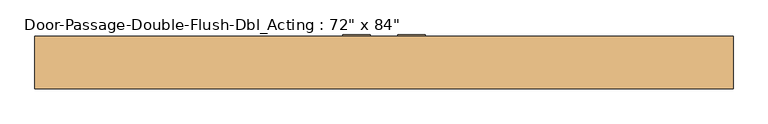
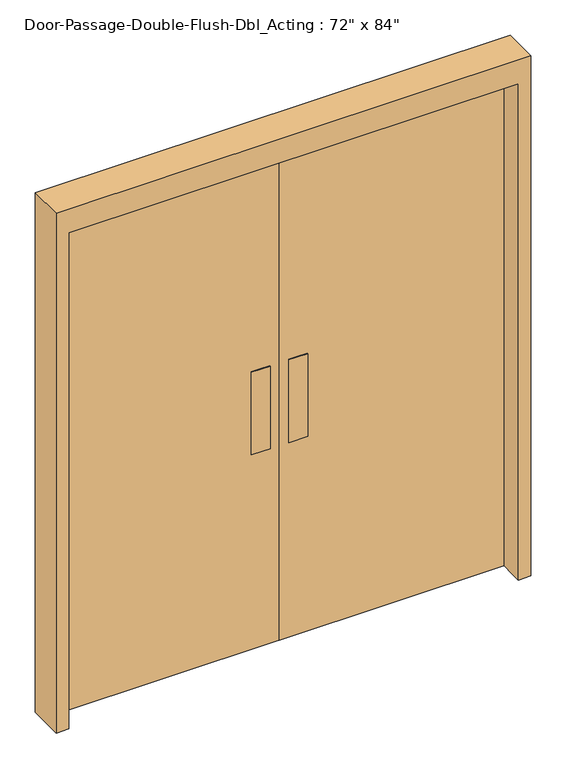
"""IFC4 building model written with IfcOpenShell, lengths in millimetres: door geometry."""

from ifc_helpers import new_model, si_unit, frame, origin, origin_with_axes, place, context, project, spatial, polyline, outline, extrude, source, transform, mapped, element, save


def door_d44e9ae0(model_context):
    return source(origin(), model_context, "Body", "SweptSolid", [
        extrude(outline(polyline([(-38.1, 34.925), (-114.3, 34.925), (-114.3, 38.1), (-38.1, 38.1), (-38.1, 34.925)])), frame((0.0, 0.0, 838.2), z_axis=(0.0, 0.0, 1.0), x_axis=(1.0, 0.0, 0.0)), (0.0, 0.0, 1.0), 355.6),
        extrude(outline(polyline([(-38.1, 85.725), (-38.1, 82.55), (-114.3, 82.55), (-114.3, 85.725), (-38.1, 85.725)])), frame((0.0, 0.0, 838.2), z_axis=(0.0, 0.0, 1.0), x_axis=(1.0, 0.0, 0.0)), (0.0, 0.0, 1.0), 355.6),
        extrude(outline(polyline([(38.1, 34.925), (38.1, 38.1), (114.3, 38.1), (114.3, 34.925), (38.1, 34.925)])), frame((0.0, 0.0, 838.2), z_axis=(0.0, 0.0, 1.0), x_axis=(1.0, 0.0, 0.0)), (0.0, 0.0, 1.0), 355.6),
        extrude(outline(polyline([(38.1, 85.725), (114.3, 85.725), (114.3, 82.55), (38.1, 82.55), (38.1, 85.725)])), frame((0.0, 0.0, 838.2), z_axis=(0.0, 0.0, 1.0), x_axis=(1.0, 0.0, 0.0)), (0.0, 0.0, 1.0), 355.6),
        extrude(outline(polyline([(0.0, 914.4), (0.0, 965.2), (2235.2, 965.2), (2235.2, -965.2), (0.0, -965.2), (0.0, -914.4), (2133.6, -914.4), (2133.6, 914.4), (0.0, 914.4)])), frame((0.0, -63.5, 0.0), z_axis=(0.0, 1.0, 0.0), x_axis=(0.0, 0.0, 1.0)), (0.0, 0.0, 1.0), 146.05),
        extrude(outline(polyline([(914.4, 38.1), (1.5875, 38.1), (1.5875, 82.55), (914.4, 82.55), (914.4, 38.1)])), origin_with_axes(), (0.0, 0.0, 1.0), 2133.6),
        extrude(outline(polyline([(-1.5875, 38.1), (-914.4, 38.1), (-914.4, 82.55), (-1.5875, 82.55), (-1.5875, 38.1)])), origin_with_axes(), (0.0, 0.0, 1.0), 2133.6),
    ])


if __name__ == "__main__":
    model = new_model("IFC4")
    model_context = context("Model", 3, world=origin())
    ifc_project = project(units=[si_unit("LENGTHUNIT", "METRE", prefix="MILLI")], contexts=[model_context])
    site = spatial("IfcSite", under=ifc_project)
    building = spatial("IfcBuilding", under=site)
    placement = place(None, origin())
    door_shape = door_d44e9ae0(model_context)
    element("IfcDoor", 1, ObjectType="Door-Passage-Double-Flush-Dbl_Acting : 72\" x 84\"", at=placement, inside=building, context=model_context, shape_type="MappedRepresentation", body=[
        mapped(door_shape, transform((0.0, 0.0, 0.0), x_axis=(1.0, 0.0, 0.0), y_axis=(0.0, 1.0, 0.0), z_axis=(0.0, 0.0, 1.0))),
    ])
    save(model, "model.ifc")

# Revit data of these elements
# Type "Door-Passage-Double-Flush-Dbl_Acting : 72\" x 84\""
#   Type Mark = "22"
#   Fire Rating = "--"
#   Assembly Code = "B2030200"
#   Analytic Construction = "Metal"
#   W = 3' - 0"
#   Thickness = 0' - 1 3/4"
#   Thermal Resistance (R) = 1.5338 (h·ft²·°F)/BTU
#   Swing Angle [instance default] = 90.00°
#   Strike Height = 3' - 4"
#   Single Panel Width = 3' - 0"
#   Rough Width [instance default] = 6' - 4"
#   Rough Height [instance default] = 7' - 4"
#   MF Opening Height [instance default] = 0' - 4"
#   MF Opening Width [instance default] = 0' - 4"
#   Inset Calculate [instance default] = 0' - 4"
#   Masonry Inset [instance default] = 0' - 1"
#   Height = 7' - 0"
#   Width = 6' - 0"
#   Heat Transfer Coefficient (U) = 0.6520 BTU/(h·ft²·°F)
#   Masonry Frame Depth = 0' - 5 3/4"
#   Masonry Frame [instance default] = yes
#   Function = 1
#   Dry Wall Frame [instance default] = no
#   Panel Material = Metal - Paint Finish - Brindle
#   Frame Material = Metal - Paint Finish - Grey
#   Door Handle Material = Aluminium
#   Visual Light Transmittance = 0
#   Solar Heat Gain Coefficient = 0
#   Wall Closure = (empty or 0)
# Element 1 (IfcDoor, "Door-Passage-Double-Flush-Dbl_Acting : 72\" x 84\"")
#   Materials on its faces: "Aluminium", "Metal - Paint Finish - Grey", "Metal - Paint Finish - Brindle"
# Materials
#   "Metal - Paint Finish - Brindle": class "Paint", colour RGB 164 133 98, transparency 0, Cost = 0
#   "Metal - Paint Finish - Grey": class "Paint", colour RGB 104 104 104, transparency 0, Cost = 0
#   "Aluminium": class "Metal", colour RGB 244 244 244, transparency 0, Description = "Aluminum 6061", Cost = 0
